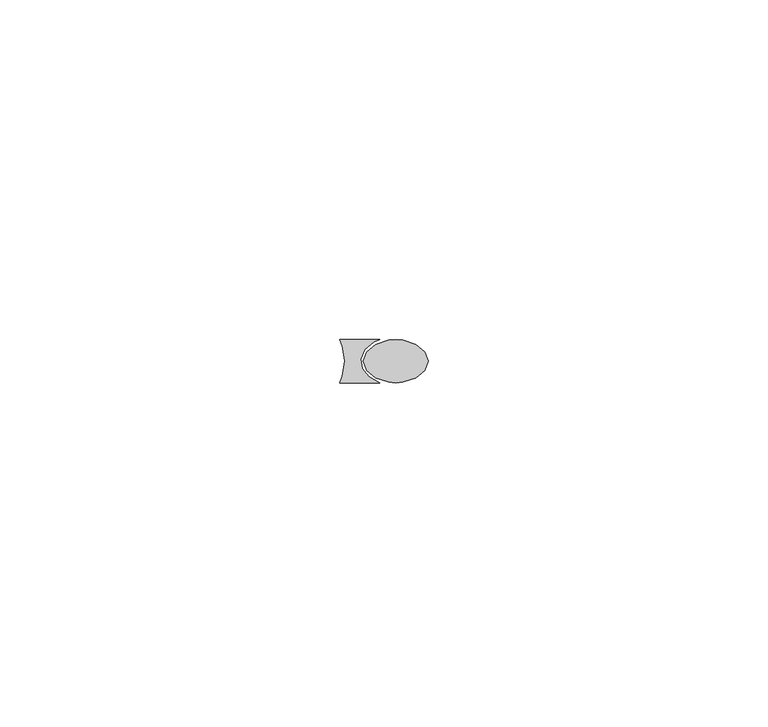
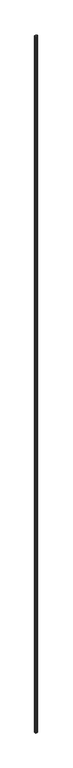
"""IFC4 building model written with IfcOpenShell, lengths in millimetres: proxy geometry, Generic Models 11:Generic Models 1:306267:Generic Models 1:306267 : Generic Models 11:Generic Models 1:306267:300405:Generic Models 1:306267:Generic Models 1:306267 : Generic Models 11:Generic Models 1:306267:300405 : Generic Models 11:Generic Models 1:306267:Generic Models 1:306267 : Generic Models 11:Generic Models 1:306267:300405:6 : Generic Models 11:Generic Models 1:306267:Generic Models 1:306267 : Generic Models 11:Generic Models 1:306267:300405:Generic Models 1:306267:Generic Models 1:306267 : Generic Models 11:Generic Models 1:306267:300405 : Generic Models 11:Generic Models 1:306267:Generic Models 1:306267 : Generic Models 11:Generic Models 1:306267:300405:300182."""

from ifc_helpers import new_model, si_unit, origin, origin_with_axes, place, context, project, spatial, polyline, outline, extrude, source, transform, mapped, element, save


def generic_models_11434219(model_context):
    return source(origin(), model_context, "Body", "SweptSolid", [
        extrude(outline(polyline([(593722.9775794, -578999.3138032), (593724.2990734, -578998.2090691), (593726.2086877, -578997.595988), (593727.2684436, -578997.5163841), (593728.3281996, -578997.595988), (593730.2378138, -578998.2090691), (593731.5593078, -578999.3138032), (593732.0309436, -579000.6913841), (593731.5593078, -579002.068965), (593730.2378138, -579003.173699), (593728.3281996, -579003.7867802), (593727.2684436, -579003.8663841), (593726.2086877, -579003.7867802), (593724.2990734, -579003.173699), (593722.9775794, -579002.068965), (593722.5059436, -579000.6913841), (593722.9775794, -578999.3138032)])), origin_with_axes(), (0.0, 0.0, 1.0), 3695.7),
        extrude(outline(polyline([(593719.4141325, -579002.9006209), (593719.7278186, -579000.6913841), (593719.4141325, -578998.4821473), (593719.0367239, -578997.5163841), (593724.904816, -578997.5163841), (593724.0445351, -578997.9027017), (593722.7349599, -578998.9861871), (593722.1346064, -579000.3364349), (593722.3373943, -579001.7422111), (593723.3115993, -579002.9835952), (593724.904816, -579003.8663841), (593719.0367239, -579003.8663841), (593719.4141325, -579002.9006209)])), origin_with_axes(), (0.0, 0.0, 1.0), 3695.7),
    ])


if __name__ == "__main__":
    model = new_model("IFC4")
    model_context = context("Model", 3, world=origin())
    ifc_project = project(units=[si_unit("LENGTHUNIT", "METRE", prefix="MILLI")], contexts=[model_context])
    site = spatial("IfcSite", under=ifc_project)
    building = spatial("IfcBuilding", under=site)
    placement = place(None, origin())
    generic_models_shape = generic_models_11434219(model_context)
    element("IfcBuildingElementProxy", 1, Name="Generic Models 11:Generic Models 1:306267:Generic Models 1:306267 : Generic Models 11:Generic Models 1:306267:300405:Generic Models 1:306267:Generic Models 1:306267 : Generic Models 11:Generic Models 1:306267:300405 : Generic Models 11:Generic Models 1:306267:Generic Models 1:306267 : Generic Models 11:Generic Models 1:306267:300405:6 : Generic Models 11:Generic Models 1:306267:Generic Models 1:306267 : Generic Models 11:Generic Models 1:306267:300405:Generic Models 1:306267:Generic Models 1:306267 : Generic Models 11:Generic Models 1:306267:300405 : Generic Models 11:Generic Models 1:306267:Generic Models 1:306267 : Generic Models 11:Generic Models 1:306267:300405:300182", ObjectType="Generic Models 11:Generic Models 1:306267:Generic Models 1:306267 : Generic Models 11:Generic Models 1:306267:300405:Generic Models 1:306267:Generic Models 1:306267 : Generic Models 11:Generic Models 1:306267:300405 : Generic Models 11:Generic Models 1:306267:Generic Models 1:306267 : Generic Models 11:Generic Models 1:306267:300405:6 : Generic Models 11:Generic Models 1:306267:Generic Models 1:306267 : Generic Models 11:Generic Models 1:306267:300405:Generic Models 1:306267:Generic Models 1:306267 : Generic Models 11:Generic Models 1:306267:300405 : Generic Models 11:Generic Models 1:306267:Generic Models 1:306267 : Generic Models 11:Generic Models 1:306267:300405:300182", at=placement, inside=building, context=model_context, shape_type="MappedRepresentation", body=[
        mapped(generic_models_shape, transform((0.0, 0.0, 0.0), x_axis=(1.0, 0.0, 0.0), y_axis=(0.0, 1.0, 0.0), z_axis=(0.0, 0.0, 1.0))),
    ])
    save(model, "model.ifc")

# Revit data of these elements
# Type "Generic Models 11:Generic Models 1:306267:Generic Models 1:306267 : Generic Models 11:Generic Models 1:306267:300405:Generic Models 1:306267:Generic Models 1:306267 : Generic Models 11:Generic Models 1:306267:300405 : Generic Models 11:Generic Models 1:306267:Generic Models 1:306267 : Generic Models 11:Generic Models 1:306267:300405:6 : Generic Models 11:Generic Models 1:306267:Generic Models 1:306267 : Generic Models 11:Generic Models 1:306267:300405:Generic Models 1:306267:Generic Models 1:306267 : Generic Models 11:Generic Models 1:306267:300405 : Generic Models 11:Generic Models 1:306267:Generic Models 1:306267 : Generic Models 11:Generic Models 1:306267:300405:300182"
#   NameOverride = "Generic Models 11:Generic Models 1:306267:Generic Models 1:306267 : Generic Models 11:Generic Models 1:306267:300405:Generic Models 1:306267:Generic Models 1:306267 : Generic Models 11:Generic Models 1:306267:300405 : Generic Models 11:Generic Models 1:306267:Generic Models 1:306267 : Generic Models 11:Generic Models 1:306267:300405:300182"
#   ObjectTypeOverride = "Generic Models 1:306267:Generic Models 1:306267 : Generic Models 11:Generic Models 1:306267:300405 : Generic Models 11:Generic Models 1:306267:Generic Models 1:306267 : Generic Models 11:Generic Models 1:306267:300405"
#   Reference = "Generic Models 1"
#   Tag = "300182"
# Element 1 (IfcBuildingElementProxy, "Generic Models 11:Generic Models 1:306267:Generic Models 1:306267 : Generic Models 11:Generic Models 1:306267:300405:Generic Models 1:306267:Generic Models 1:306267 : Generic Models 11:Generic Models 1:306267:300405 : Generic Models 11:Generic Models 1:306267:Generic Models 1:306267 : Generic Models 11:Generic Models 1:306267:300405:6 : Generic Models 11:Generic Models 1:306267:Generic Models 1:306267 : Generic Models 11:Generic Models 1:306267:300405:Generic Models 1:306267:Generic Models 1:306267 : Generic Models 11:Generic Models 1:306267:300405 : Generic Models 11:Generic Models 1:306267:Generic Models 1:306267 : Generic Models 11:Generic Models 1:306267:300405:300182")
#   Materials on its faces: "SEALANT & BACKER ROD, IF NECESSARY"
# Materials
#   "SEALANT & BACKER ROD, IF NECESSARY": class "Unassigned", colour RGB 120 120 120, transparency 0, Cost = 0
